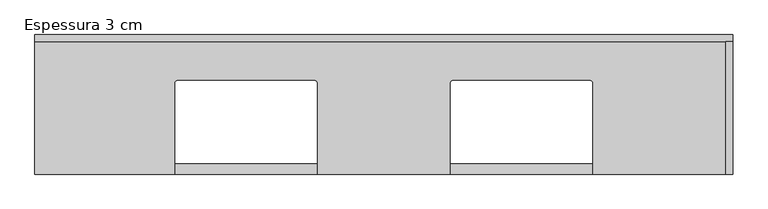
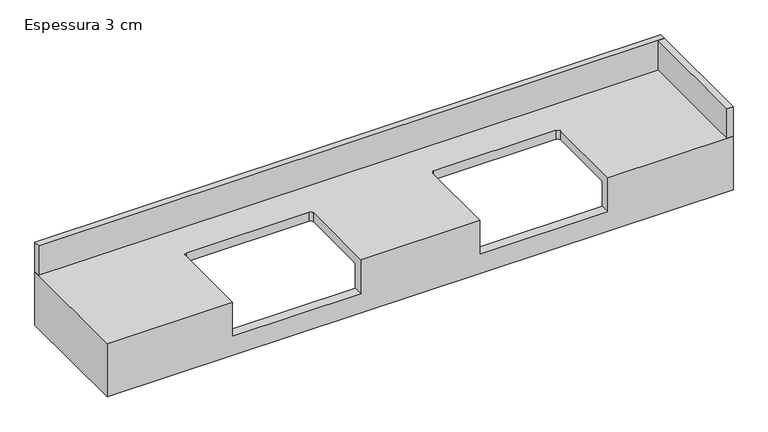
"""IFC4 building model written with IfcOpenShell, lengths in millimetres: furniture geometry, CC_BANCADA BANHEIRO COM DUAS CUBAS_CANTO RETO : Espessura 3 cm."""

from ifc_helpers import new_model, si_unit, frame, origin, place, context, project, spatial, polyline, circle_curve, outline, extrude, source, transform, mapped, element, save
from ifc_brep_helpers import plane_surface, revolved_surface, advanced_brep


def espessura_3_cm_7ff6149e(model_context):
    return source(origin(), model_context, "Body", "SolidModel", [
        advanced_brep(
        [(750.0, 300.0, 860.0), (-1250.0, 300.0, 860.0), (-1250.0, -100.0, 860.0), (-850.0, -100.0, 860.0), (-850.0, 160.0, 860.0), (-840.0, 170.0, 860.0), (-450.0, 170.0, 860.0), (-440.0, 160.0, 860.0), (-440.0, -100.0, 860.0), (-60.0, -100.0, 860.0), (-60.0, 160.0, 860.0), (-50.0, 170.0, 860.0), (340.0, 170.0, 860.0), (350.0, 160.0, 860.0), (350.0, -100.0, 860.0), (750.0, -100.0, 860.0), (750.0, 300.0, 680.0), (720.0, 300.0, 680.0), (720.0, 300.0, 830.0), (-1220.0, 300.0, 830.0), (-1220.0, 300.0, 680.0), (-1250.0, 300.0, 680.0), (-1250.0, -100.0, 680.0), (750.0, -100.0, 680.0), (350.0, -100.0, 745.0), (-60.0, -100.0, 745.0), (-440.0, -100.0, 745.0), (-850.0, -100.0, 745.0), (720.0, -70.0, 830.0), (350.0, -70.0, 830.0), (350.0, 160.0, 830.0), (340.0, 170.0, 830.0), (-50.0, 170.0, 830.0), (-60.0, 160.0, 830.0), (-60.0, -70.0, 830.0), (-440.0, -70.0, 830.0), (-440.0, 160.0, 830.0), (-450.0, 170.0, 830.0), (-840.0, 170.0, 830.0), (-850.0, 160.0, 830.0), (-850.0, -70.0, 830.0), (-1220.0, -70.0, 830.0), (-1220.0, -70.0, 680.0), (-850.0, -70.0, 745.0), (-440.0, -70.0, 745.0), (-60.0, -70.0, 745.0), (350.0, -70.0, 745.0), (720.0, -70.0, 680.0)],
        [
            (0, 1),
            (1, 2),
            (2, 3),
            (3, 4),
            (4, 5, circle_curve(frame((-840.0, 160.0, 860.0), z_axis=(0.0, 0.0, -1.0), x_axis=(0.0, 1.0, 0.0)), 10.0)),
            (5, 6),
            (6, 7, circle_curve(frame((-450.0, 160.0, 860.0), z_axis=(0.0, 0.0, -1.0), x_axis=(0.0, 1.0, 0.0)), 10.0)),
            (7, 8),
            (8, 9),
            (9, 10),
            (10, 11, circle_curve(frame((-50.0, 160.0, 860.0), z_axis=(0.0, 0.0, -1.0), x_axis=(0.0, 1.0, 0.0)), 10.0)),
            (11, 12),
            (12, 13, circle_curve(frame((340.0, 160.0, 860.0), z_axis=(0.0, 0.0, -1.0), x_axis=(0.0, 1.0, 0.0)), 10.0)),
            (13, 14),
            (14, 15),
            (15, 0),
            (0, 16),
            (16, 17),
            (17, 18),
            (18, 19),
            (19, 20),
            (20, 21),
            (21, 1),
            (21, 22),
            (22, 2),
            (22, 23),
            (23, 15),
            (14, 24),
            (24, 25),
            (25, 9),
            (8, 26),
            (26, 27),
            (27, 3),
            (23, 16),
            (18, 28),
            (28, 29),
            (29, 30),
            (30, 31, circle_curve(frame((340.0, 160.0, 830.0), z_axis=(0.0, 0.0, 1.0), x_axis=(0.0, 1.0, 0.0)), 10.0)),
            (31, 32),
            (32, 33, circle_curve(frame((-50.0, 160.0, 830.0), z_axis=(0.0, 0.0, 1.0), x_axis=(0.0, 1.0, 0.0)), 10.0)),
            (33, 34),
            (34, 35),
            (35, 36),
            (36, 37, circle_curve(frame((-450.0, 160.0, 830.0), z_axis=(0.0, 0.0, 1.0), x_axis=(0.0, 1.0, 0.0)), 10.0)),
            (37, 38),
            (38, 39, circle_curve(frame((-840.0, 160.0, 830.0), z_axis=(0.0, 0.0, 1.0), x_axis=(0.0, 1.0, 0.0)), 10.0)),
            (39, 40),
            (40, 41),
            (41, 19),
            (41, 42),
            (42, 20),
            (40, 43),
            (43, 44),
            (44, 35),
            (34, 45),
            (45, 46),
            (46, 29),
            (28, 47),
            (47, 42),
            (17, 47),
            (5, 38),
            (37, 6),
            (26, 44),
            (43, 27),
            (4, 39),
            (7, 36),
            (24, 46),
            (45, 25),
            (11, 32),
            (31, 12),
            (10, 33),
            (13, 30),
        ],
        [
            plane_surface(frame((-1250.0, 300.0, 860.0), z_axis=(0.0, 0.0, 1.0), x_axis=(-1.0, 0.0, 0.0))),
            plane_surface(frame((750.0, 300.0, 860.0), z_axis=(0.0, 1.0, 0.0), x_axis=(0.0, 0.0, -1.0))),
            plane_surface(frame((-1250.0, 300.0, 860.0), z_axis=(-1.0, 0.0, 0.0), x_axis=(0.0, 0.0, -1.0))),
            plane_surface(frame((-1250.0, -100.0, 860.0), z_axis=(0.0, -1.0, 0.0), x_axis=(0.0, 0.0, -1.0))),
            plane_surface(frame((750.0, -100.0, 860.0), z_axis=(1.0, 0.0, 0.0), x_axis=(0.0, 0.0, -1.0))),
            plane_surface(frame((-1220.0, 300.0, 830.0), z_axis=(0.0, 0.0, -1.0), x_axis=(-1.0, 0.0, 0.0))),
            plane_surface(frame((-1220.0, 300.0, 830.0), z_axis=(1.0, 0.0, 0.0), x_axis=(0.0, 0.0, -1.0))),
            plane_surface(frame((-1220.0, -70.0, 830.0), z_axis=(0.0, 1.0, 0.0), x_axis=(0.0, 0.0, -1.0))),
            plane_surface(frame((720.0, -70.0, 830.0), z_axis=(-1.0, 0.0, 0.0), x_axis=(0.0, 0.0, -1.0))),
            plane_surface(frame((750.0, -100.0, 680.0), z_axis=(0.0, 0.0, -1.0), x_axis=(0.0, 1.0, 0.0))),
            plane_surface(frame((-840.0, 170.0, 745.0), z_axis=(0.0, -1.0, 0.0), x_axis=(0.0, 0.0, 1.0))),
            plane_surface(frame((-450.0, 170.0, 745.0), z_axis=(0.0, 0.0, 1.0), x_axis=(1.0, 0.0, 0.0))),
            revolved_surface(polyline([(-840.0, 170.0, 830.0), (-840.0, 170.0, 860.0)]), (-840.0, 160.0, 900.0), (0.0, 0.0, -1.0)),
            plane_surface(frame((-850.0, -230.0, 745.0), z_axis=(1.0, 0.0, 0.0), x_axis=(0.0, 0.0, 1.0))),
            plane_surface(frame((-440.0, 160.0, 745.0), z_axis=(-1.0, 0.0, 0.0), x_axis=(0.0, 0.0, 1.0))),
            revolved_surface(polyline([(-450.0, 170.0, 830.0), (-450.0, 170.0, 860.0)]), (-450.0, 160.0, 900.0), (0.0, 0.0, -1.0)),
            plane_surface(frame((340.0, 170.0, 745.0), z_axis=(0.0, 0.0, 1.0), x_axis=(1.0, 0.0, 0.0))),
            plane_surface(frame((-50.0, 170.0, 745.0), z_axis=(0.0, -1.0, 0.0), x_axis=(0.0, 0.0, 1.0))),
            revolved_surface(polyline([(-50.0, 170.0, 830.0), (-50.0, 170.0, 860.0)]), (-50.0, 160.0, 900.0), (0.0, 0.0, -1.0)),
            plane_surface(frame((-60.0, -230.0, 745.0), z_axis=(1.0, 0.0, 0.0), x_axis=(0.0, 0.0, 1.0))),
            plane_surface(frame((350.0, 160.0, 745.0), z_axis=(-1.0, 0.0, 0.0), x_axis=(0.0, 0.0, 1.0))),
            revolved_surface(polyline([(340.0, 170.0, 830.0), (340.0, 170.0, 860.0)]), (340.0, 160.0, 900.0), (0.0, 0.0, -1.0)),
        ],
        [
            (0, [[1, 2, 3, 4, 5, 6, 7, 8, 9, 10, 11, 12, 13, 14, 15, 16]]),
            (1, [[-1, 17, 18, 19, 20, 21, 22, 23]]),
            (2, [[-2, -23, 24, 25]]),
            (3, [[-3, -25, 26, 27, -15, 28, 29, 30, -9, 31, 32, 33]]),
            (4, [[-16, -27, 34, -17]]),
            (5, [[35, 36, 37, 38, 39, 40, 41, 42, 43, 44, 45, 46, 47, 48, 49, -20]]),
            (6, [[-49, 50, 51, -21]]),
            (7, [[-48, 52, 53, 54, -42, 55, 56, 57, -36, 58, 59, -50]]),
            (8, [[-35, -19, 60, -58]]),
            (9, [[-18, -34, -26, -24, -22, -51, -59, -60]]),
            (10, [[-6, 61, -45, 62]]),
            (11, [[-32, 63, -53, 64]]),
            (12, [[-5, 65, -46, -61]]),
            (13, [[-4, -33, -64, -52, -47, -65]]),
            (14, [[-8, 66, -43, -54, -63, -31]]),
            (15, [[-7, -62, -44, -66]]),
            (16, [[-29, 67, -56, 68]]),
            (17, [[-12, 69, -39, 70]]),
            (18, [[-11, 71, -40, -69]]),
            (19, [[-10, -30, -68, -55, -41, -71]]),
            (20, [[-14, 72, -37, -57, -67, -28]]),
            (21, [[-13, -70, -38, -72]]),
        ],
    ),
        extrude(outline(polyline([(730.0, 280.0), (750.0, 280.0), (750.0, -100.0), (730.0, -100.0), (730.0, 280.0)])), frame((0.0, 0.0, 860.0), z_axis=(0.0, 0.0, 1.0), x_axis=(1.0, 0.0, 0.0)), (0.0, 0.0, 1.0), 100.0),
        extrude(outline(polyline([(750.0, 300.0), (750.0, 280.0), (-1250.0, 280.0), (-1250.0, 300.0), (750.0, 300.0)])), frame((0.0, 0.0, 860.0), z_axis=(0.0, 0.0, 1.0), x_axis=(1.0, 0.0, 0.0)), (0.0, 0.0, 1.0), 100.0),
    ])


if __name__ == "__main__":
    model = new_model("IFC4")
    model_context = context("Model", 3, world=origin())
    ifc_project = project(units=[si_unit("LENGTHUNIT", "METRE", prefix="MILLI")], contexts=[model_context])
    site = spatial("IfcSite", under=ifc_project)
    building = spatial("IfcBuilding", under=site)
    placement = place(None, origin())
    espessura_3_cm_shape = espessura_3_cm_7ff6149e(model_context)
    element("IfcFurniture", 1, ObjectType="CC_BANCADA BANHEIRO COM DUAS CUBAS_CANTO RETO : Espessura 3 cm", at=placement, inside=building, context=model_context, shape_type="MappedRepresentation", body=[
        mapped(espessura_3_cm_shape, transform((0.0, 0.0, 0.0), x_axis=(1.0, 0.0, 0.0), y_axis=(0.0, 1.0, 0.0), z_axis=(0.0, 0.0, 1.0))),
    ])
    save(model, "model.ifc")

# Revit data of these elements
# Type "CC_BANCADA BANHEIRO COM DUAS CUBAS_CANTO RETO : Espessura 3 cm"
#   Uso HS [instance default] = ""
#   h TESTEIRA AUX [instance default] = 0.15 m
#   Altura testeira [instance default] = 0.15 m
#   Altura rodapia [instance default] = 0.10 m
#   Espessura rodapia [instance default] = 0.02 m
#   Prof/2 [instance default] = 0.20 m
#   Offset cuba direita [instance default] = 0.40 m
#   Offset cuba esquerda [instance default] = 0.40 m
#   Depth [instance default] = 2.00 m
#   Width [instance default] = 0.40 m
#   Espessura bancada = 0.03 m
#   Comprimento [instance default] = 2.00 m
#   Height [instance default] = 0.86 m
#   Testeira [instance default] = yes
#   Rodapia fundo [instance default] = no
#   Rodapia esquerda [instance default] = no
#   Rodapia direita [instance default] = no
#   Material porta-toalha [instance default] = .CROMADO
#   Material hidráulico [instance default] = .CROMADO
#   Material cuba [instance default] = .PORCELANA BRANCA
#   Material bancada [instance default] = .GRANITO_BRANCO_ITAUNAS
#   Assembly Code = ""
# Element 1 (IfcFurniture, "CC_BANCADA BANHEIRO COM DUAS CUBAS_CANTO RETO : Espessura 3 cm")
#   Uso HS = "SUÍTE MASTER"
#   Rodapia fundo = yes
#   Rodapia direita = yes
#   Materials on its faces: ".GRANITO_BRANCO_ITAUNAS"
# Materials
#   ".CROMADO": class "CC_METAIS", colour RGB 211 223 226, transparency 0, Cost = 0
#   ".PORCELANA BRANCA": class "CC_PORCELANA", colour RGB 230 230 230, transparency 0, Cost = 0
#   ".GRANITO_BRANCO_ITAUNAS": class ".CC_PEDRA REVEST.", colour RGB 202 195 174, transparency 0, Description = "Revestimento em granito", Cost = 0
